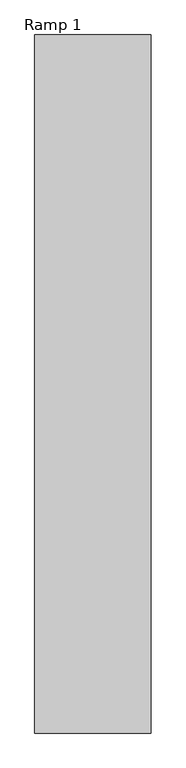
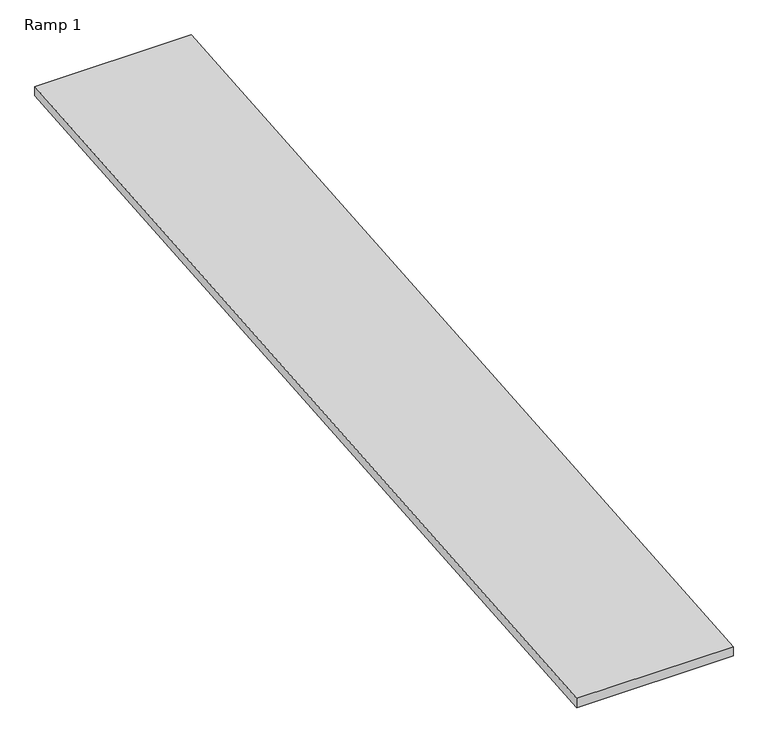
"""IFC4 building model written with IfcOpenShell, lengths in millimetres: ramp geometry, Ramp 1."""

from ifc_helpers import new_model, si_unit, frame, origin, place, context, project, spatial, polyline, outline, extrude, source, transform, mapped, element, save


def ramp_1_51a07ffc(model_context):
    return source(origin(), model_context, "Body", "SweptSolid", [
        extrude(outline(polyline([(-8058.4292912, 0.0), (-858.4292912, 600.0), (-858.4292912, 524.7400339), (-8058.4292912, -75.2599661), (-8058.4292912, 0.0)])), frame((-599.8488078, 0.0, 0.0), z_axis=(1.0, 0.0, 0.0), x_axis=(0.0, 1.0, 0.0)), (0.0, 0.0, 1.0), 1200.0),
    ])


if __name__ == "__main__":
    model = new_model("IFC4")
    model_context = context("Model", 3, world=origin())
    ifc_project = project(units=[si_unit("LENGTHUNIT", "METRE", prefix="MILLI")], contexts=[model_context])
    site = spatial("IfcSite", under=ifc_project)
    building = spatial("IfcBuilding", under=site)
    placement = place(None, origin())
    ramp_1_shape = ramp_1_51a07ffc(model_context)
    element("IfcRamp", 1, ObjectType="Ramp 1", at=placement, inside=building, context=model_context, shape_type="MappedRepresentation", body=[
        mapped(ramp_1_shape, transform((0.0, 0.0, 0.0), x_axis=(1.0, 0.0, 0.0), y_axis=(0.0, 1.0, 0.0), z_axis=(0.0, 0.0, 1.0))),
    ])
    save(model, "model.ifc")
